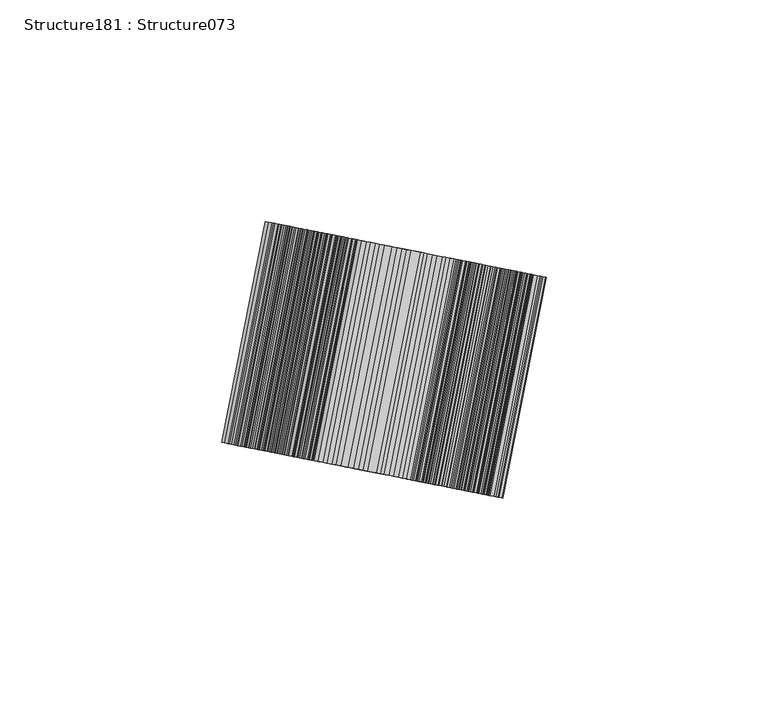
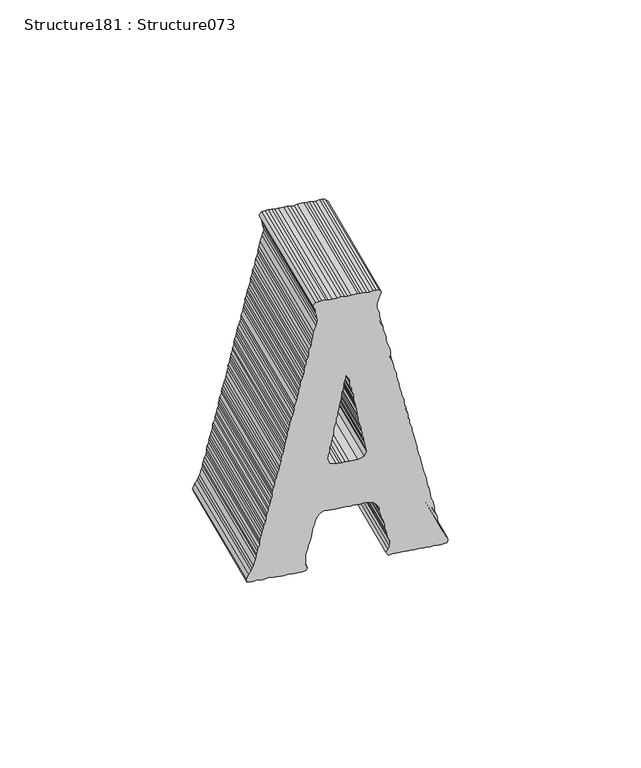
"""IFC4 building model written with IfcOpenShell, lengths in millimetres: proxy geometry, Structure181 : Structure073."""

import ifcopenshell
import ifcopenshell.guid

model = None  # the IFC model being written
_history = None  # IfcOwnerHistory: only IFC2X3 demands one
_inside = {}  # id of a spatial element -> (the spatial element, [elements in it])
_under = {}  # id of a project, library or spatial element -> (it, [spatial elements below it])
_declared = {}  # id of a project -> (the project, [libraries it declares])
_typed = {}  # id of a type object -> (the type object, [elements of that type])
_made_of = {}  # id of a material, layer set ... -> (it, [elements and type objects made of it])


def new_model(schema):
    """Start an empty IFC model of exactly this schema.

    Asked for "IFC4X3", IfcOpenShell would pick the latest addendum, in which some entities
    have other attributes; the version numbers below select the first issue.
    IFC2X3 requires an IfcOwnerHistory on every rooted entity: one is made here for all.
    """
    global model, _history
    if schema == "IFC4X3":
        model = ifcopenshell.file(schema_version=(4, 3, 0, 0))
    else:
        model = ifcopenshell.file(schema=schema)
    _inside.clear()
    _under.clear()
    _declared.clear()
    _typed.clear()
    _made_of.clear()
    _history = None
    if model.schema == "IFC2X3":
        org = make("IfcOrganization", Name="unknown")
        user = make(
            "IfcPersonAndOrganization",
            ThePerson=make("IfcPerson", FamilyName="unknown"),
            TheOrganization=org,
        )
        app = make(
            "IfcApplication",
            ApplicationDeveloper=org,
            Version="unknown",
            ApplicationFullName="unknown",
            ApplicationIdentifier="unknown",
        )
        _history = make(
            "IfcOwnerHistory",
            OwningUser=user,
            OwningApplication=app,
            ChangeAction="ADDED",
            CreationDate=0,
        )
    return model


def make(cls, **values):
    """One entity of the class cls with the attributes given. An attribute that is None is left unset."""
    return model.create_entity(
        cls, **{name: value for name, value in values.items() if value is not None}
    )


def rooted(cls, **values):
    """An entity with a GlobalId (a new one), such as an element, a storey or a relation."""
    return make(cls, GlobalId=ifcopenshell.guid.new(), OwnerHistory=_history, **values)


def si_unit(unit_type, name, prefix=None):
    """IfcSIUnit, for example si_unit("LENGTHUNIT", "METRE", prefix="MILLI")."""
    return make("IfcSIUnit", UnitType=unit_type, Prefix=prefix, Name=name)


def assignment(units):
    """IfcUnitAssignment: the units of a project."""
    return None if units is None else make("IfcUnitAssignment", Units=units)


def point(xyz):
    """IfcCartesianPoint."""
    return None if xyz is None else make("IfcCartesianPoint", Coordinates=xyz)


def direction(xyz):
    """IfcDirection."""
    return None if xyz is None else make("IfcDirection", DirectionRatios=xyz)


def frame(location, z_axis=None, x_axis=None):
    """IfcAxis2Placement3D, a coordinate frame: its origin and axes. An axis left out is left unset."""
    return make(
        "IfcAxis2Placement3D",
        Location=point(location),
        Axis=direction(z_axis),
        RefDirection=direction(x_axis),
    )


def origin():
    """The frame at (0, 0, 0) with its axes left unset."""
    return frame((0.0, 0.0, 0.0))


def place(relative_to, where):
    """IfcLocalPlacement: puts the frame where relative to a parent placement (None: the world)."""
    return make(
        "IfcLocalPlacement", PlacementRelTo=relative_to, RelativePlacement=where
    )


def context(
    kind, dimensions, precision=None, world=None, true_north=None, identifier=None
):
    """IfcGeometricRepresentationContext, for example the 3D "Model" context."""
    return make(
        "IfcGeometricRepresentationContext",
        ContextIdentifier=identifier,
        ContextType=kind,
        CoordinateSpaceDimension=dimensions,
        Precision=precision,
        WorldCoordinateSystem=world,
        TrueNorth=true_north,
    )


def project(units=None, contexts=None):
    """IfcProject with its units and contexts."""
    return rooted(
        "IfcProject",
        Name="project",
        RepresentationContexts=contexts,
        UnitsInContext=assignment(units),
    )


def spatial(cls, under=None, at=None, **own):
    """A site, building, storey or space (cls), placed at a placement, below another one or the project."""
    s = rooted(cls, ObjectPlacement=at, **own)
    if under is not None:
        _under.setdefault(under.id(), (under, []))[1].append(s)
    return s


def polyline(points):
    """IfcPolyline through the points."""
    return make("IfcPolyline", Points=[point(p) for p in points])


def outline(outer, holes=None, kind="AREA"):
    """IfcArbitraryClosedProfileDef: a profile drawn as a closed curve; with holes, ...WithVoids."""
    if holes is None:
        return make("IfcArbitraryClosedProfileDef", ProfileType=kind, OuterCurve=outer)
    return make(
        "IfcArbitraryProfileDefWithVoids",
        ProfileType=kind,
        OuterCurve=outer,
        InnerCurves=holes,
    )


def extrude(swept, where, along, depth):
    """IfcExtrudedAreaSolid: the profile swept, set in the frame where, extruded along a direction by depth."""
    return make(
        "IfcExtrudedAreaSolid",
        SweptArea=swept,
        Position=where,
        ExtrudedDirection=direction(along),
        Depth=depth,
    )


def shape(context_of_items, identifier, shape_type, items):
    """IfcShapeRepresentation: the items that make up one representation, for example the "Body"."""
    return make(
        "IfcShapeRepresentation",
        ContextOfItems=context_of_items,
        RepresentationIdentifier=identifier,
        RepresentationType=shape_type,
        Items=items,
    )


def source(mapping_origin, context_of_items, identifier, shape_type, items):
    """IfcRepresentationMap: a shape defined once, which mapped items show again and again."""
    return make(
        "IfcRepresentationMap",
        MappingOrigin=mapping_origin,
        MappedRepresentation=shape(context_of_items, identifier, shape_type, items),
    )


def transform(
    local_origin,
    x_axis=None,
    y_axis=None,
    z_axis=None,
    scale=None,
    scale2=None,
    scale3=None,
    uniform=True,
):
    """IfcCartesianTransformationOperator3D, or its non-uniform kind. x_axis, y_axis, z_axis: its Axis1, 2, 3."""
    if uniform:
        return make(
            "IfcCartesianTransformationOperator3D",
            Axis1=direction(x_axis),
            Axis2=direction(y_axis),
            LocalOrigin=point(local_origin),
            Scale=scale,
            Axis3=direction(z_axis),
        )
    return make(
        "IfcCartesianTransformationOperator3DnonUniform",
        Axis1=direction(x_axis),
        Axis2=direction(y_axis),
        LocalOrigin=point(local_origin),
        Scale=scale,
        Axis3=direction(z_axis),
        Scale2=scale2,
        Scale3=scale3,
    )


def mapped(mapping_source, mapping_target):
    """IfcMappedItem: shows the shape of a source again, moved by a transform."""
    return make(
        "IfcMappedItem", MappingSource=mapping_source, MappingTarget=mapping_target
    )


def made_of(thing, what):
    """Note that an element or type object is made of a material, layer set ...; save() writes the relation."""
    if what is not None:
        _made_of.setdefault(what.id(), (what, []))[1].append(thing)
    return thing


def element(
    cls,
    number,
    at=None,
    inside=None,
    cuts=None,
    type_object=None,
    material=None,
    context=None,
    identifier="Body",
    shape_type=None,
    held_by="IfcProductDefinitionShape",
    body=None,
    shapes=None,
    **own,
):
    """One element of the class cls, such as IfcWall. Its Tag is "e" and its number.

    at: its placement. inside: the storey or other place that contains it. cuts: it is an
    opening in that element (IfcRelVoidsElement). A single representation is given by context,
    identifier, shape_type and body (its items); several are given by shapes. held_by: the class
    of the entity that holds the representations. save() writes the other relations.
    """
    e = rooted(cls, Tag="e%d" % number, ObjectPlacement=at, **own)
    if body is not None:
        shapes = [shape(context, identifier, shape_type, body)]
    if shapes is not None:
        e.Representation = make(held_by, Representations=shapes)
    if inside is not None:
        _inside.setdefault(inside.id(), (inside, []))[1].append(e)
    if cuts is not None:
        rooted(
            "IfcRelVoidsElement", RelatingBuildingElement=cuts, RelatedOpeningElement=e
        )
    if type_object is not None:
        _typed.setdefault(type_object.id(), (type_object, []))[1].append(e)
    return made_of(e, material)


def aggregate(whole, parts):
    """IfcRelAggregates: a whole, such as a stair, and the parts it consists of."""
    return rooted("IfcRelAggregates", RelatingObject=whole, RelatedObjects=parts)


def save(model, path):
    """Write the relations noted so far, then the file.

    IfcRelAggregates (storeys below a building ...), IfcRelContainedInSpatialStructure (elements
    in a storey), IfcRelDefinesByType, IfcRelAssociatesMaterial and IfcRelDeclares: one each for
    every whole, place, type object, material and project.
    """
    for whole, parts in _under.values():
        aggregate(whole, parts)
    for where, things in _inside.values():
        rooted(
            "IfcRelContainedInSpatialStructure",
            RelatedElements=things,
            RelatingStructure=where,
        )
    for kind, things in _typed.values():
        rooted("IfcRelDefinesByType", RelatedObjects=things, RelatingType=kind)
    for what, things in _made_of.values():
        rooted("IfcRelAssociatesMaterial", RelatedObjects=things, RelatingMaterial=what)
    for by, libraries in _declared.values():
        rooted("IfcRelDeclares", RelatingContext=by, RelatedDefinitions=libraries)
    model.write(path)


def structure181_structure073_ac0dd930(model_context):
    return source(origin(), model_context, "Body", "SweptSolid", [
        extrude(outline(polyline([(0.9094651, 0.0), (2.0811665, -0.5191352), (2.9906316, -0.6525661), (4.1562841, -0.7810156), (5.1991801, -1.166364), (5.9748585, -1.299795), (7.1504738, -1.6901249), (8.1894559, -1.6901249), (9.3551083, -2.0808106), (10.2645735, -2.3426911), (11.4362748, -2.5995901), (12.3453841, -2.8564891), (13.3818755, -2.9849386), (14.1582655, -3.3756242), (15.4626861, -3.5090551), (16.3721513, -3.5090551), (17.5385154, -3.7709355), (19.491944, -4.413183), (20.2718921, -4.6750635), (21.3101626, -4.9369439), (22.3470097, -4.9369439), (23.2561191, -5.1991801), (24.4278204, -5.58951), (25.4700048, -5.9748585), (26.6363689, -5.9748585), (27.4124031, -6.3651884), (28.7175354, -6.6270688), (30.535754, -7.0177545), (31.5743802, -7.146204), (32.7400327, -7.4080845), (33.6555467, -7.7934329), (35.4741211, -7.7934329), (36.5102567, -7.536534), (37.5492387, -7.279635), (38.3288311, -6.8843236), (39.3671015, -6.3651884), (40.4099976, -7.279635), (40.5395145, -8.1837628), (40.5395145, -9.0982094), (40.2826155, -10.2645734), (40.2826155, -11.3021323), (40.5395145, -12.4734778), (40.4099976, -13.2541376), (40.5395145, -14.1636027), (40.5395145, -16.2390762), (40.2826155, -17.2819722), (40.2826155, -18.3198868), (40.5395145, -19.4858951), (40.4099976, -20.662222), (40.4099976, -22.3473656), (40.2826155, -23.5187111), (40.5395145, -24.422839), (40.5395145, -25.5991659), (40.4099976, -26.5036497), (40.2826155, -27.6696579), (39.2382962, -28.455655), (38.3288311, -27.9315383), (37.4197218, -27.6696579), (36.6397736, -27.5461898), (35.4741211, -27.2843094), (33.5199809, -26.8939795), (32.6112274, -27.1558599), (31.4448633, -27.4177403), (29.3636968, -28.1937746), (27.545834, -28.455655), (26.5089869, -28.712554), (25.3372855, -28.8459848), (24.2943895, -29.1078652), (23.2561191, -29.6216632), (21.3101626, -29.7504686), (20.2718921, -30.012349), (19.491944, -30.5361098), (18.3202426, -30.5361098), (17.2816164, -30.9214583), (16.3721513, -31.1783572), (15.3356599, -31.1783572), (14.1582655, -31.4405935), (13.1253323, -31.8309234), (12.2158672, -32.2212533), (11.4362748, -32.3546842), (10.2645735, -32.4831337), (9.3551083, -32.8684822), (8.1894559, -32.8684822), (7.1504738, -33.259168), (6.2374505, -33.3925988), (5.0714422, -33.6494978), (3.2475306, -34.2967267), (2.0811665, -34.2967267), (1.1720572, -34.5586072), (0.1334309, -34.8208434), (-1.0382704, -35.3396228), (-1.8178628, -35.4730536), (-2.8568449, -35.7299526), (-3.8990293, -35.8633836), (-5.0653934, -36.2487321), (-5.8471206, -36.5109683), (-7.0166871, -36.5109683), (-8.1826954, -36.9012982), (-8.9644226, -37.0297477), (-10.1364798, -37.4200777), (-11.1690572, -37.5535086), (-12.2115974, -37.6769765), (-12.9915456, -37.938857), (-14.03373, -38.3295427), (-15.3292552, -38.4579922), (-16.3678815, -38.7198726), (-18.1861001, -39.1102026), (-19.3581573, -39.3671016), (-20.2672666, -39.7577873), (-21.4371888, -40.0196676), (-22.2189161, -40.2765666), (-23.1223323, -40.538447), (-24.1648726, -40.538447), (-25.465735, -41.052245), (-26.5025822, -41.3144813), (-27.4173846, -41.4479122), (-28.4560108, -41.4479122), (-29.235959, -41.7048112), (-30.5311284, -42.095141), (-31.3110766, -42.228572), (-32.3536168, -42.6139205), (-33.5214042, -42.6139205), (-34.4308693, -43.1330557), (-35.3399786, -43.3949361), (-36.37647, -43.3949361), (-37.5424783, -43.6568165), (-38.7202285, -44.0471464), (-39.6236447, -44.3040454), (-40.405372, -44.5613002), (-41.5752942, -44.6947311), (-42.6139205, -45.085061), (-43.7856218, -45.3469415), (-44.8221132, -45.3469415), (-45.7372714, -45.475391), (-46.6406876, -45.9941703), (-47.812389, -46.2514251), (-48.8510152, -46.5133055), (-49.7601245, -46.5133055), (-50.6731478, -46.9036354), (-52.8777823, -47.5508644), (-53.7929405, -47.9415501), (-54.5689747, -48.33188), (-55.738897, -49.1125398), (-57.5532016, -49.7601245), (-58.4665807, -49.4982441), (-58.5957419, -48.2034305), (-58.4665807, -47.4273963), (-58.3331498, -46.2514251), (-58.5957419, -45.2135105), (-58.5957419, -44.0471464), (-58.3331498, -43.0046062), (-58.3331498, -42.095141), (-58.4665807, -41.052245), (-58.4665807, -40.1481171), (-58.5957419, -38.8483221), (-58.5957419, -37.938857), (-58.4665807, -36.9012982), (-58.3331498, -35.7299526), (-58.5957419, -34.8208434), (-58.5957419, -31.8309234), (-58.3331498, -30.6645593), (-57.4297336, -30.1407985), (-56.6480063, -30.5361098), (-55.6115149, -30.7930088), (-53.3972734, -30.7930088), (-52.3586471, -30.7930088), (-51.4495378, -30.5361098), (-50.6731478, -30.1407985), (-49.3683714, -30.012349), (-48.4592621, -29.7504686), (-47.5497969, -29.3597828), (-46.6406876, -29.1078652), (-45.6038405, -28.8459848), (-43.2661308, -28.5841045), (-41.5752942, -27.9315383), (-40.2762109, -27.6696579), (-38.9767716, -27.0274104), (-38.1950444, -26.1129639), (-37.4190102, -24.6847194), (-37.6759092, -23.6471606), (-37.6759092, -21.5667057), (-37.5424783, -20.2669108), (-37.5424783, -17.5438526), (-37.6759092, -16.3675256), (-37.4190102, -15.4633978), (-37.5424783, -14.4205017), (-37.6759092, -13.3829429), (-37.5424783, -12.4734778), (-37.4190102, -11.1736828), (-37.6759092, -10.3930229), (-38.0676623, -8.836329), (-38.8476105, -8.0553133), (-40.2762109, -7.0177545), (-41.4422191, -7.0177545), (-42.6139205, -6.7558741), (-44.561656, -6.2367389), (-45.3472973, -5.7179595), (-46.5133056, -5.4560791), (-47.2932538, -5.3276296), (-48.33188, -5.3276296), (-49.3683714, -4.8084944), (-50.4126907, -4.6750635), (-51.4495378, -4.546614), (-52.3586471, -4.1612655), (-53.6595096, -3.7709355), (-55.3489229, -3.899385), (-56.6480063, -4.289715), (-57.2966585, -4.9369439), (-58.5957419, -4.1612655), (-58.4665807, -2.9849386), (-58.3331498, -1.9473797), (-58.3331498, 0.1284495), (-58.4665807, 1.1660084), (-58.4665807, 2.2089043), (-58.3331498, 3.1180137), (-58.4665807, 4.0324602), (-58.4665807, 5.3272738), (-58.3331498, 6.1029522), (-58.4665807, 7.4027472), (-58.3331498, 8.1837628), (-58.5957419, 9.2213217), (-58.3331498, 10.3976486), (-58.5957419, 11.5640127), (-58.4665807, 12.473122), (-58.3331498, 13.5160181), (-58.3331498, 14.5485954), (-57.2966585, 14.9442626), (-56.3875492, 14.6820263), (-55.738897, 14.0298161), (-54.5689747, 13.772917), (-53.7929405, 13.3825872), (-52.6151903, 12.8634519), (-50.6731478, 11.9543426), (-49.8875066, 11.6924622), (-48.5941162, 11.5640127), (-47.5497969, 11.3017765), (-46.6406876, 11.0448775), (-45.8646534, 10.6545476), (-44.561656, 10.5260981), (-42.6139205, 10.2642177), (-41.4422192, 9.8738877), (-40.5384471, 9.4832021), (-39.6236447, 9.2213217), (-38.4576364, 9.0928722), (-37.4190102, 8.9694041), (-36.5059869, 8.8359732), (-35.6004358, 8.3171937), (-34.2956593, 8.1837628), (-33.3922431, 8.0549575), (-32.3536168, 7.926508), (-31.4405935, 7.5361781), (-30.4019673, 7.1458483), (-29.235959, 6.8889493), (-27.5447666, 6.6270688), (-26.3752002, 6.2363831), (-25.203143, 6.1029522), (-24.4235506, 5.8460532), (-23.3849244, 5.4607047), (-22.4793732, 5.3272738), (-21.3037579, 4.9369439), (-20.2672666, 4.9369439), (-19.3581573, 4.6747077), (-18.319531, 4.4178087), (-17.1474738, 4.1559283), (-15.2018732, 3.6371488), (-14.1632469, 3.3802498), (-13.1207067, 3.3802498), (-12.2115974, 2.9895642), (-11.3024881, 2.5992343), (-10.0012698, 2.5992343), (-9.2270147, 2.0804548), (-8.1826954, 2.0804548), (-7.0166871, 1.9520054), (-5.9745027, 1.4278887), (-5.0653934, 1.4278887), (-4.1619771, 0.9091093), (-2.8568449, 0.7756784), (-1.9473797, 0.7756784), (-0.7817273, 0.2618804), (0.0, 0.0), (0.9094651, 0.0)]), holes=[polyline([(-20.9137838, -13.9017224), (-20.9137838, -16.8916423), (-20.7903157, -18.0576506), (-21.0472147, -19.2289961), (-20.7903157, -20.1384613), (-20.9137838, -21.0475705), (-20.2672666, -22.9945944), (-18.5817672, -23.6471606), (-17.2809048, -23.3852802), (-16.3678815, -23.1280253), (-15.4623303, -22.8661449), (-14.1632469, -22.9945944), (-13.2480888, -22.4807964), (-12.2115974, -22.3473656), (-11.3024881, -22.2189161), (-10.393023, -21.8285862), (-9.3508386, -21.6951552), (-8.3122123, -21.6951552), (-7.146204, -21.5667057), (-6.3644768, -21.17602), (-5.3276296, -20.919121), (-4.2854452, -20.919121), (-3.117302, -20.4003417), (-1.9473797, -20.4003417), (-1.0382704, -20.0100118), (-0.2561874, -19.8765808), (1.0389821, -19.7477755), (2.0811665, -19.4858951), (3.1180136, -19.2289961), (4.0274787, -19.1005466), (5.0714422, -19.1005466), (6.1082894, -18.5817672), (7.0177545, -18.4483363), (8.1894559, -18.4483363), (9.2216774, -18.0576506), (10.1368356, -17.7957702), (11.0463007, -17.7957702), (10.1368356, -17.1535227), (9.0928721, -16.7582113), (8.056025, -16.6297618), (6.8900167, -16.6297618), (6.1082894, -16.1106267), (4.9365881, -15.9771958), (3.1180136, -15.4633978), (1.8189302, -15.3299668), (0.9094651, -15.2015174), (0.0, -14.9396369), (-1.0382704, -14.8108316), (-2.2078369, -14.4205017), (-4.2854452, -14.2870708), (-5.3276296, -14.0351532), (-6.3644768, -13.9017224), (-8.1826954, -13.5113924), (-9.2270147, -12.9922572), (-10.2638619, -12.9922572), (-11.1690572, -12.7303768), (-12.3446725, -12.6019273), (-13.1207067, -12.2165788), (-14.286715, -12.2165788), (-15.4623303, -11.8212675), (-17.2809048, -11.5640127), (-18.5817672, -11.3021323), (-20.1377496, -12.0831479), (-20.9137838, -13.9017224)])]), frame((-2748.3458068, 235013.9109386, 444.9951864), z_axis=(0.19466222296394123, 0.9808703374813295, 0.0), x_axis=(0.0, 0.0, 1.0)), (0.0, 0.0, 1.0), 50.8),
    ])


if __name__ == "__main__":
    model = new_model("IFC4")
    model_context = context("Model", 3, world=origin())
    ifc_project = project(units=[si_unit("LENGTHUNIT", "METRE", prefix="MILLI")], contexts=[model_context])
    site = spatial("IfcSite", under=ifc_project)
    building = spatial("IfcBuilding", under=site)
    placement = place(None, origin())
    structure181_structure073_shape = structure181_structure073_ac0dd930(model_context)
    element("IfcBuildingElementProxy", 1, Name="Structure181 : Structure073", ObjectType="Structure181 : Structure073", at=placement, inside=building, context=model_context, shape_type="MappedRepresentation", body=[
        mapped(structure181_structure073_shape, transform((0.0, 0.0, 0.0), x_axis=(1.0, 0.0, 0.0), y_axis=(0.0, 1.0, 0.0), z_axis=(0.0, 0.0, 1.0))),
    ])
    save(model, "model.ifc")

# Revit data of these elements
# Type "Structure181 : Structure073"
#   NameOverride = "Structure073"
# Element 1 (IfcBuildingElementProxy, "Structure181 : Structure073")
#   Materials on its faces: "BRUSHED ALUMINUM LETTERING"
# Materials
#   "BRUSHED ALUMINUM LETTERING": class "Unassigned", colour RGB 169 181 186, transparency 0, Cost = 0
